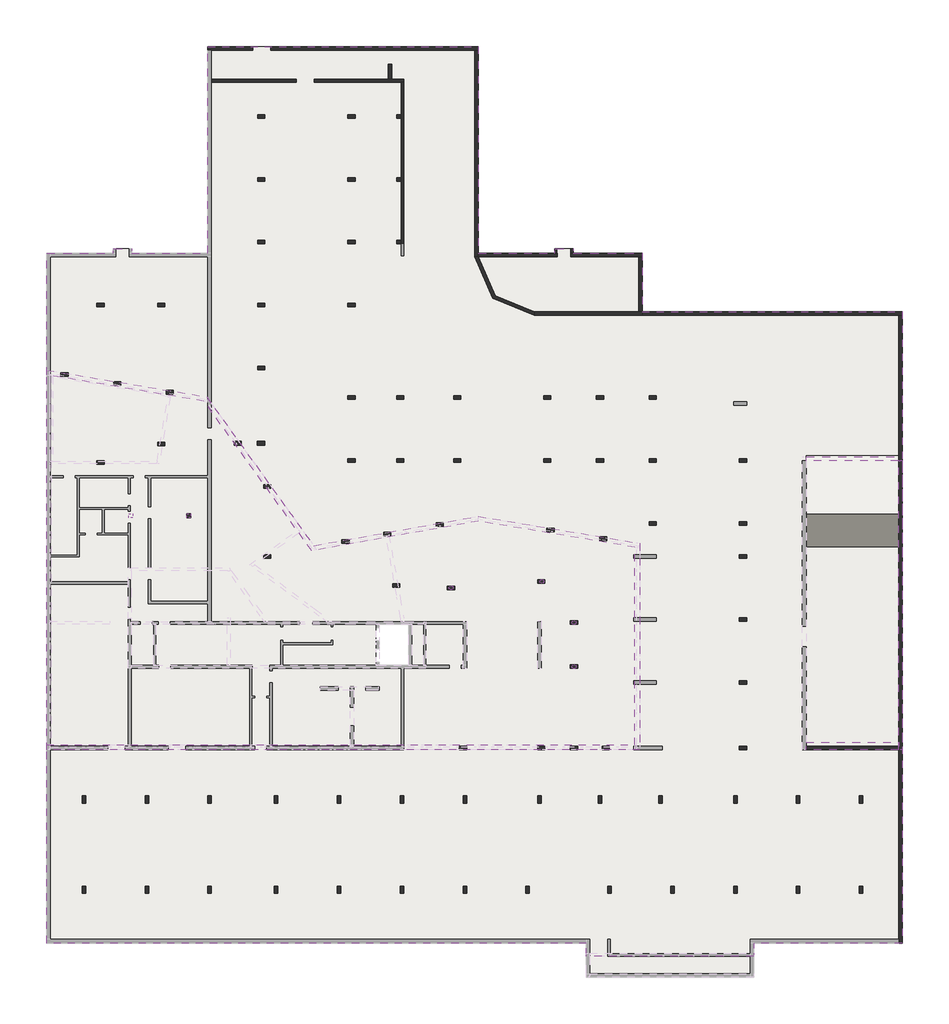
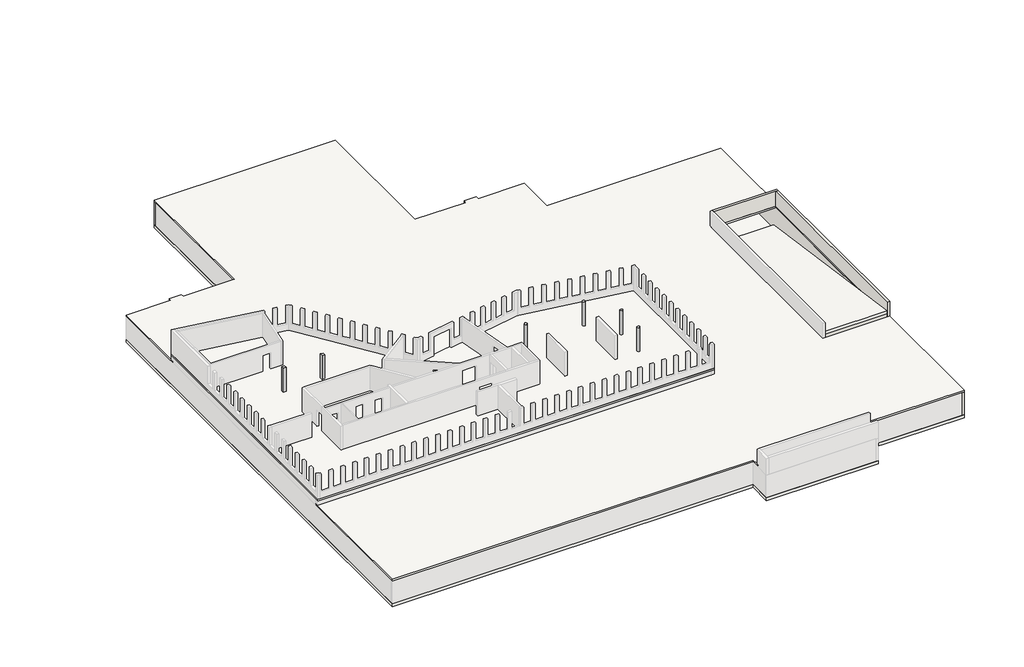
# One storey, part 4 of 4: 89 columns, 17 walls, 4 slabs.
# Revit data of these elements (continued)
# Type "5dki STB-Stützen rund : 5dki Stütze rund ø35cm C40/50"
#   cpiFitMatchKey = "5D-KI-STB-OB-ST-RUN"
#   cpiComponentType = "Column"
#   5d Materialgüte = "C40/50"
#   Radius = 0.175 m
#   Durchmesser = 0.350 m
#   5dki Bewehrung Stab kg pro m3 = 0
#   5dki Sichtbeton SB3/SB4 [instance default] = no
#   Structural Material = 5d Beton - Stahlbeton
#   Assembly Code = ""
# Type "5dki STB-Stützen rechteckig : 5dki Stütze recht. 35x35cm C35/45"
#   cpiFitMatchKey = "5D-KI-STB-OB-ST-REC"
#   cpiComponentType = "Column"
#   5d Materialgüte = "C35/45"
#   Tiefe = 0.350 m
#   Breite = 0.350 m
#   5dki Bewehrung Stab kg pro m3 = 0
#   5dki Sichtbeton SB3/SB4 [instance default] = no
#   Structural Material = 5d Beton - Stahlbeton
#   Assembly Code = ""
# Type "5dki STB-Stützen rechteckig : 5dki Stütze recht. 60x30 cm C35/45"
#   cpiFitMatchKey = "5D-KI-STB-OB-ST-REC"
#   cpiComponentType = "Column"
#   5d Materialgüte = "C35/45"
#   Tiefe = 0.300 m
#   Breite = 0.600 m
#   5dki Bewehrung Stab kg pro m3 = 0
#   5dki Sichtbeton SB3/SB4 [instance default] = no
#   Structural Material = 5d Beton - Stahlbeton
#   Assembly Code = ""
# Type "5dki Bodenplatte 40cm C30/37"
#   cpiComponentType = "Foundation_Slab"
#   cpiFitMatchKey = "5D-KI-STB-OB-BoPla"
#   5d Materialgüte = "C30/37"
#   5dki Bewehrung Stab kg pro m3 = 0
#   5dki Bewehrung Liste kg pro m3 = 0
#   5dki Bewehrung Matte kg pro m3 = 0
#   5dki WU = no
#   Layers, outside or top first: 0.400 m "5d Beton - Stahlbeton" (function 1)
# Type "5dki Bodenplatte 40cm C40/50"
#   cpiComponentType = "Foundation_Slab"
#   cpiFitMatchKey = "5D-KI-STB-OB-BoPla"
#   5d Materialgüte = "C40/50"
#   5dki Bewehrung Stab kg pro m3 = 0
#   5dki Bewehrung Liste kg pro m3 = 0
#   5dki Bewehrung Matte kg pro m3 = 0
#   5dki WU = no
#   Layers, outside or top first: 0.400 m "5d Beton - Stahlbeton" (function 1)
# Type "5dki Decke Ortbeton 25cm C30/37"
#   cpiComponentType = "Slab"
#   cpiFitMatchKey = "5D-KI-STB-OB-DE"
#   5d Materialgüte = "C30/37"
#   Function = 0
#   5dki WU = no
#   Layers, outside or top first: 0.250 m "5d Beton - Stahlbeton" (function 1)
# Type "5dki STB-Wand 30cm WU C35/45"
#   Type Comments = ""
#   Description = ""
#   cpiComponentType = "Wall"
#   cpiFitMatchKey = "5D-KI-STB-OB-W"
#   5d Materialgüte = "C35/45"
#   Filter Tragend / Nichttragend = yes
#   5dki WU = yes
#   Layers, outside or top first: 0.300 m "5d Beton - Stahlbeton WU" (function 1)
# Type "5dki STB-Wand 20cm WU C30/37"
#   Type Comments = ""
#   Description = ""
#   cpiComponentType = "Wall"
#   cpiFitMatchKey = "5D-KI-STB-OB-W"
#   5d Materialgüte = "C30/37"
#   Filter Tragend / Nichttragend = yes
#   5dki WU = yes
#   Layers, outside or top first: 0.200 m "5d Beton - Stahlbeton WU" (function 1)
# Type "5dki Überzug 60cm C30/37"
#   Type Comments = ""
#   Description = ""
#   cpiComponentType = "Beam"
#   cpiFitMatchKey = "5D-KI-STB-OB-TR-UEZ"
#   5d Materialgüte = "C30/37"
#   Filter Tragend / Nichttragend = yes
#   Layers, outside or top first: 0.600 m "5d Beton - Stahlbeton" (function 1)
# Type "5dki STB-Wand 20cm C25/30"
#   Type Comments = ""
#   Description = ""
#   cpiComponentType = "Wall"
#   cpiFitMatchKey = "5D-KI-STB-OB-W"
#   5d Materialgüte = "C25/30"
#   Filter Tragend / Nichttragend = yes
#   5dki WU = no
#   Layers, outside or top first: 0.200 m "5d Beton - Stahlbeton" (function 1)
# Type "5dki STB-Wand 25cm C30/37"
#   Type Comments = ""
#   Description = ""
#   cpiComponentType = "Wall"
#   cpiFitMatchKey = "5D-KI-STB-OB-W"
#   5d Materialgüte = "C30/37"
#   Filter Tragend / Nichttragend = yes
#   5dki WU = no
#   Layers, outside or top first: 0.250 m "5d Beton - Stahlbeton" (function 1)
# Type "5dki STB-Wand 30cm C30/37"
#   Type Comments = ""
#   Description = ""
#   cpiComponentType = "Wall"
#   cpiFitMatchKey = "5D-KI-STB-OB-W"
#   5d Materialgüte = "C30/37"
#   Filter Tragend / Nichttragend = yes
#   5dki WU = no
#   Layers, outside or top first: 0.300 m "5d Beton - Stahlbeton" (function 1)
# Element 1 (IfcColumn, "5dki STB-Stützen rund : 5dki Stütze rund ø35cm C40/50")
#   Comments = ""
#   000_080_030_Geschoß = "00_EG"
#   5dki Sichtbeton SB3/SB4 = no
#   Phase Created = Neu
#   Materials on its faces: "5d Beton - Stahlbeton"
# Element 2 (IfcColumn, "5dki STB-Stützen rechteckig : 5dki Stütze recht. 35x35cm C35/45")
#   Comments = ""
#   000_080_030_Geschoß = "00_EG"
#   5dki Sichtbeton SB3/SB4 = no
#   Phase Created = Neu
#   Materials on its faces: "5d Beton - Stahlbeton"
# Element 3 (IfcColumn, "5dki STB-Stützen rechteckig : 5dki Stütze recht. 35x35cm C35/45")
#   000_080_030_Geschoß = "00_EG"
#   5dki Sichtbeton SB3/SB4 = no
#   Phase Created = Neu
#   Materials on its faces: "5d Beton - Stahlbeton"
# Elements 4, 5, 6 (IfcColumn, "5dki STB-Stützen rund : 5dki Stütze rund ø35cm C40/50")
#   000_080_030_Geschoß = "00_EG"
#   5dki Sichtbeton SB3/SB4 = no
#   Phase Created = Neu
#   Materials on its faces: "5d Beton - Stahlbeton"
# Elements 7, 8, 9, 11, 12, 13, 14, 15, 16, 17, 18, 19, 20, 21, 22, 23, 24, 25, 26, 27, 28, 29, 30, 31, 32, 33, 34, 35, 36, 37, 38, 39, 40, 41, 42, 43, 44, 45, 46, 47, 48, 49, 50, 51, 52, 53, 54, 55, 56, 57, 58, 59, 60, 61, 62, 63, 64, 65, 66, 67, 68, 69, 70, 71, 72, 73, 74, 75, 76, 77, 78, 79, 80, 81, 82, 83, 84, 85, 86, 87, 88, 89 (IfcColumn, "5dki STB-Stützen rechteckig : 5dki Stütze recht. 60x30 cm C35/45")
#   Comments = ""
#   000_080_030_Geschoß = "01_UG"
#   5dki Sichtbeton SB3/SB4 = no
#   Phase Created = Neu
#   Materials on its faces: "5d Beton - Stahlbeton"
# Element 10 (IfcColumn, "5dki STB-Stützen rechteckig : 5dki Stütze recht. 35x35cm C35/45")
#   Comments = ""
#   000_080_030_Geschoß = "01_UG"
#   5dki Sichtbeton SB3/SB4 = no
#   Phase Created = Neu
#   Materials on its faces: "5d Beton - Stahlbeton"
# Element 90 (IfcSlab, "5dki Bodenplatte 40cm C30/37")
#   000_080_030_Geschoß = "01_UG"
#   Height Offset From Level = 0.000 m
#   built-in parameter 1001954 = 1
#   Phase Created = Neu
#   Materials on its faces: "5d Beton - Stahlbeton"
# Element 91 (IfcSlab, "5dki Bodenplatte 40cm C40/50")
#   Comments = ""
#   000_080_030_Geschoß = "02_FU"
#   Height Offset From Level = 0.000 m
#   built-in parameter 1001954 = 1
#   Phase Created = Neu
#   Materials on its faces: "5d Beton - Stahlbeton"
# Element 92 (IfcSlab, "5dki Decke Ortbeton 25cm C30/37")
#   000_080_030_Geschoß = "01_UG"
#   built-in parameter 1001955 = -0.165462 (stored number, unit not read)
#   Height Offset From Level = 0.000 m
#   built-in parameter 1001954 = 1
#   Phase Created = Neu
#   Materials on its faces: "5d Beton - Stahlbeton"
# Element 93 (IfcSlab, "5dki Decke Ortbeton 25cm C30/37")
#   000_080_030_Geschoß = "01_UG"
#   Height Offset From Level = 0.000 m
#   Phase Created = Neu
#   Materials on its faces: "5d Beton - Stahlbeton"
# Elements 94, 95, 96, 97 (IfcWall, "5dki STB-Wand 30cm WU C35/45")
#   Comments = ""
#   000_080_030_Geschoß = "01_UG"
#   Top Offset = 0.000 m
#   Base Offset = 0.000 m
#   wall height = 3.000 m
#   Phase Created = Neu
#   Base Constraint = 02_FU_OKRD_-4,20
#   Top Constraint = 01_UG_UKRD_-1,20
#   Materials on its faces: "5d Beton - Stahlbeton WU"
# Elements 98, 99 (IfcWall, "5dki STB-Wand 30cm WU C35/45")
#   000_080_030_Geschoß = "01_UG"
#   Top Offset = 0.000 m
#   Base Offset = 0.000 m
#   wall height = 3.000 m
#   Phase Created = Neu
#   Base Constraint = 02_FU_OKRD_-4,20
#   Top Constraint = 01_UG_UKRD_-1,20
#   Materials on its faces: "5d Beton - Stahlbeton WU"
# Element 100 (IfcWall, "5dki STB-Wand 20cm WU C30/37")
#   Comments = ""
#   000_080_030_Geschoß = "01_UG"
#   Top Offset = 0.000 m
#   Base Offset = 0.000 m
#   wall height = 3.000 m
#   Phase Created = Neu
#   Base Constraint = 01_UG_OKFB_-4,20
#   Top Constraint = 01_UG_UKRD_-1,20
#   Materials on its faces: "5d Beton - Stahlbeton WU"
# Element 101 (IfcWall, "5dki STB-Wand 20cm WU C30/37")
#   000_080_030_Geschoß = "01_UG"
#   Top Offset = 0.000 m
#   Base Offset = 0.000 m
#   wall height = 3.000 m
#   Phase Created = Neu
#   Base Constraint = 01_UG_OKFB_-4,20
#   Top Constraint = 01_UG_UKRD_-1,20
#   Materials on its faces: "5d Beton - Stahlbeton WU"
# Element 102 (IfcWall, "5dki Überzug 60cm C30/37")
#   Comments = ""
#   000_080_030_Geschoß = "01_UG"
#   Top Offset = 0.000 m
#   Base Offset = 0.000 m
#   wall height = 0.800 m
#   Phase Created = Neu
#   Base Constraint = 01_UG_UKRD_-1,20
#   Top Constraint = 01_UG_UKRD_-0,40
#   Materials on its faces: "5d Beton - Stahlbeton"
# Element 103 (IfcWall, "5dki STB-Wand 20cm C25/30")
#   Comments = ""
#   000_080_030_Geschoß = "01_UG"
#   Top Offset = 0.000 m
#   Base Offset = 0.000 m
#   wall height = 3.000 m
#   Phase Created = Neu
#   Base Constraint = 02_FU_OKRD_-4,20
#   Top Constraint = 01_UG_UKRD_-1,20
#   Materials on its faces: "5d Beton - Stahlbeton"
# Element 104 (IfcWall, "5dki STB-Wand 25cm C30/37")
#   Comments = ""
#   000_080_030_Geschoß = "01_UG"
#   Top Offset = 0.000 m
#   Base Offset = 0.000 m
#   wall height = 3.000 m
#   Phase Created = Neu
#   Base Constraint = 02_FU_OKRD_-4,20
#   Top Constraint = 01_UG_UKRD_-1,20
#   Materials on its faces: "5d Beton - Stahlbeton"
# Elements 105, 106 (IfcWall, "5dki STB-Wand 30cm C30/37")
#   Comments = ""
#   000_080_030_Geschoß = "01_UG"
#   Top Offset = 0.000 m
#   Base Offset = 0.000 m
#   wall height = 3.000 m
#   Phase Created = Neu
#   Base Constraint = 02_FU_OKRD_-4,20
#   Top Constraint = 01_UG_UKRD_-1,20
#   Materials on its faces: "5d Beton - Stahlbeton"
# Element 107 (IfcWall, "5dki STB-Wand 30cm C30/37")
#   Comments = ""
#   000_080_030_Geschoß = "01_UG"
#   Top Offset = 0.000 m
#   Base Offset = 0.000 m
#   Unconnected Height = 4.000 m
#   wall height = 3.000 m
#   Phase Created = Neu
#   Materials on its faces: "5d Beton - Stahlbeton"
# Element 108 (IfcWall, "5dki STB-Wand 30cm C30/37")
#   Comments = ""
#   000_080_030_Geschoß = "01_UG"
#   Top Offset = 0.000 m
#   Base Offset = 0.000 m
#   wall height = 3.000 m
#   Phase Created = Neu
#   Base Constraint = 02_FU_OKRD_-4,20
#   Top Constraint = 01_UG_UKRD_-1,20
#   Materials on its faces: "5d Beton - Stahlbeton", "5d Beton - Stahlbeton WU"
# Elements 109, 110 (IfcWall, "5dki STB-Wand 30cm C30/37")
#   Comments = ""
#   000_080_030_Geschoß = "00_EG"
#   Top Offset = 0.000 m
#   Base Offset = 0.000 m
#   wall height = 1.950 m
#   Phase Created = Neu
#   Base Constraint = 01_UG_OKRD_-0,95
#   Top Constraint = 00_EG_OKWA_1,00
#   Materials on its faces: "5d Beton - Stahlbeton"
# Materials
#   "5d Beton - Stahlbeton": class "5dki", colour RGB 200 200 200, transparency 0, Cost = 0
#   "5d Beton - Stahlbeton WU": class "5dki", colour RGB 190 205 190, transparency 0, Cost = 0
